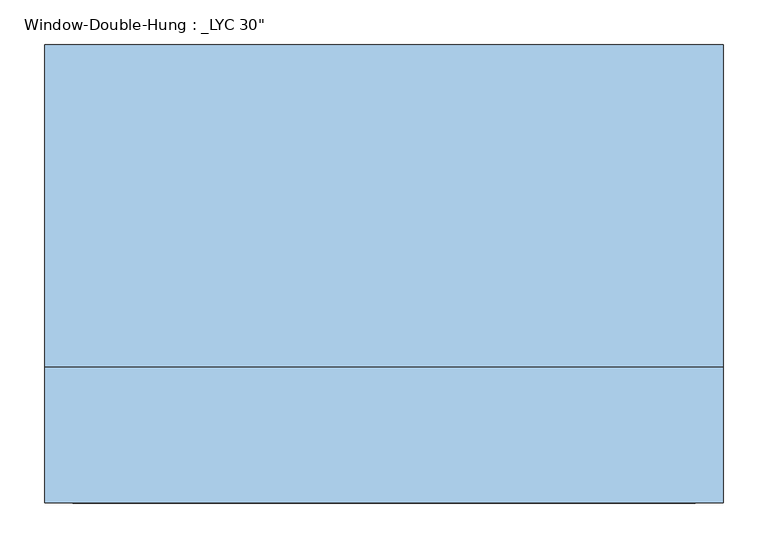
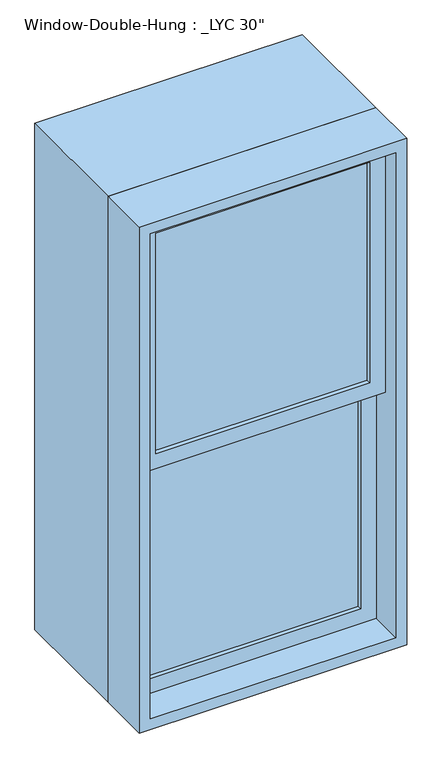
"""IFC4 building model written with IfcOpenShell, lengths in millimetres: window geometry."""

from ifc_helpers import new_model, si_unit, frame, origin, place, context, project, spatial, polyline, outline, extrude, source, transform, mapped, element, save


def window_5da76499(model_context):
    return source(origin(), model_context, "Body", "SweptSolid", [
        extrude(outline(polyline([(304.8, -158.75), (-304.8, -158.75), (-304.8, -152.4), (304.8, -152.4), (304.8, -158.75)])), frame((0.0, 0.0, 990.6), z_axis=(0.0, 0.0, 1.0), x_axis=(1.0, 0.0, 0.0)), (0.0, 0.0, 1.0), 663.575),
        extrude(outline(polyline([(-304.8, -146.05), (-304.8, -139.7), (304.8, -139.7), (304.8, -146.05), (-304.8, -146.05)])), frame((0.0, 0.0, 990.6), z_axis=(0.0, 0.0, 1.0), x_axis=(1.0, 0.0, 0.0)), (0.0, 0.0, 1.0), 663.575),
        extrude(outline(polyline([(304.8, -203.2), (-304.8, -203.2), (-304.8, -196.85), (304.8, -196.85), (304.8, -203.2)])), frame((0.0, 0.0, 1698.625), z_axis=(0.0, 0.0, 1.0), x_axis=(1.0, 0.0, 0.0)), (0.0, 0.0, 1.0), 663.575),
        extrude(outline(polyline([(-304.8, -190.5), (-304.8, -184.15), (304.8, -184.15), (304.8, -190.5), (-304.8, -190.5)])), frame((0.0, 0.0, 1698.625), z_axis=(0.0, 0.0, 1.0), x_axis=(1.0, 0.0, 0.0)), (0.0, 0.0, 1.0), 663.575),
        extrude(outline(polyline([(1698.625, 349.25), (1698.625, -349.25), (946.15, -349.25), (946.15, 349.25), (1698.625, 349.25)]), holes=[polyline([(1654.175, -304.8), (1654.175, 304.8), (990.6, 304.8), (990.6, -304.8), (1654.175, -304.8)])]), frame((0.0, -171.45, 0.0), z_axis=(0.0, 1.0, 0.0), x_axis=(0.0, 0.0, 1.0)), (0.0, 0.0, 1.0), 44.45),
        extrude(outline(polyline([(2406.65, 349.25), (2406.65, -349.25), (1654.175, -349.25), (1654.175, 349.25), (2406.65, 349.25)]), holes=[polyline([(2362.2, -304.8), (2362.2, 304.8), (1698.625, 304.8), (1698.625, -304.8), (2362.2, -304.8)])]), frame((0.0, -215.9, 0.0), z_axis=(0.0, 1.0, 0.0), x_axis=(0.0, 0.0, 1.0)), (0.0, 0.0, 1.0), 44.45),
        extrude(outline(polyline([(2438.4, 381.0), (2438.4, -381.0), (914.4, -381.0), (914.4, 381.0), (2438.4, 381.0)]), holes=[polyline([(2406.65, -349.25), (2406.65, 349.25), (946.15, 349.25), (946.15, -349.25), (2406.65, -349.25)])]), frame((0.0, -266.7, 0.0), z_axis=(0.0, 1.0, 0.0), x_axis=(0.0, 0.0, 1.0)), (0.0, 0.0, 1.0), 152.4),
        extrude(outline(polyline([(2438.4, 381.0), (2438.4, -381.0), (914.4, -381.0), (914.4, 381.0), (2438.4, 381.0)]), holes=[polyline([(2419.35, 361.95), (933.45, 361.95), (933.45, -361.95), (2419.35, -361.95), (2419.35, 361.95)])]), frame((0.0, -114.3, 0.0), z_axis=(0.0, 1.0, 0.0), x_axis=(0.0, 0.0, 1.0)), (0.0, 0.0, 1.0), 361.95),
    ])


if __name__ == "__main__":
    model = new_model("IFC4")
    model_context = context("Model", 3, world=origin())
    ifc_project = project(units=[si_unit("LENGTHUNIT", "METRE", prefix="MILLI")], contexts=[model_context])
    site = spatial("IfcSite", under=ifc_project)
    building = spatial("IfcBuilding", under=site)
    placement = place(None, origin())
    window_shape = window_5da76499(model_context)
    element("IfcWindow", 1, ObjectType="Window-Double-Hung : _LYC 30\"", at=placement, inside=building, context=model_context, shape_type="MappedRepresentation", body=[
        mapped(window_shape, transform((0.0, 0.0, 0.0), x_axis=(1.0, 0.0, 0.0), y_axis=(0.0, 1.0, 0.0), z_axis=(0.0, 0.0, 1.0))),
    ])
    save(model, "model.ifc")

# Revit data of these elements
# Type "Window-Double-Hung : _LYC 30\""
#   Type Mark = "19"
#   Fire Rating = "0.5h"
#   Assembly Code = "B2020100"
#   Wall Thickness [instance default] = 0' - 6"
#   Visual Light Transmittance = 0.9
#   Thermal Resistance (R) = 1.8146 (h·ft²·°F)/BTU
#   Solar Heat Gain Coefficient = 0.78
#   Rough Width = 2' - 6 1/2"
#   Rough Height = 5' - 0 1/2"
#   Muntin Width = 2' - 0"
#   Muntin Height = 2' - 2 1/8"
#   Interior Wall Closure [instance default] = 0' - 1 1/2"
#   Heat Transfer Coefficient (U) = 0.6496 BTU/(h·ft²·°F)
#   Frame Extension [instance default] = 0' - 2"
#   Exterior Wall Closure [instance default] = 0' - 0 1/2"
#   Extension Jamb [instance default] = 0' - 0 3/4"
#   Height = 5' - 0"
#   Width = 2' - 6"
#   Window Inset [instance default] = 0' - 0 3/4"
#   Top Muntin Visibility = yes
#   Interior Trim Visibility [instance default] = yes
#   Indicator Visibility [instance default] = yes
#   Exterior Trim Visibility [instance default] = yes
#   Extension Jamb Visibility [instance default] = yes
#   Define Thermal Properties by = 1
#   Bottom Muntin Visibility = yes
#   Muntin Pattern = Muntin Pattern_2x2 : Muntin Pattern_2x2
#   Interior Trim Material = Wood - Stained
#   Interior Trim = Trim-Window-Interior-Flat : Picture Frame
#   Interior Frame Material = Wood - Stained
#   Glass Panel Material = Glass
#   Exterior Trim Material = Clad - White
#   Exterior Trim = Trim-Window-Exterior-Flat : with Sill
#   Exterior Frame Material = Clad - White
#   Construction Type Id = ""
#   Wall Closure = (empty or 0)
#   Analytic Construction = (empty or 0)
# Element 1 (IfcWindow, "Window-Double-Hung : _LYC 30\"")
#   Wall Thickness = 1' - 7 1/2"
#   Extension Jamb = 1' - 2 1/4"
#   Materials on its faces: "Wood - Stained", "Glass", "Clad - White"
# Materials
#   "Wood - Stained": class "Wood", colour RGB 224 178 126, transparency 0, Cost = 0
#   "Glass": class "Unassigned", colour RGB 0 128 192, transparency 0.75
#   "Clad - White": class "Wood", colour RGB 242 242 238, transparency 0, Cost = 0
